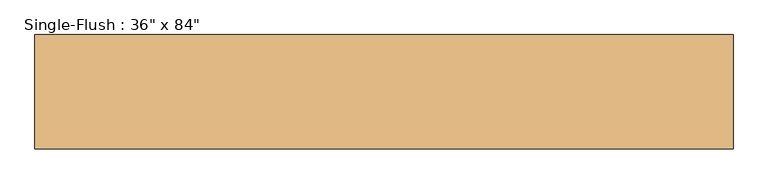
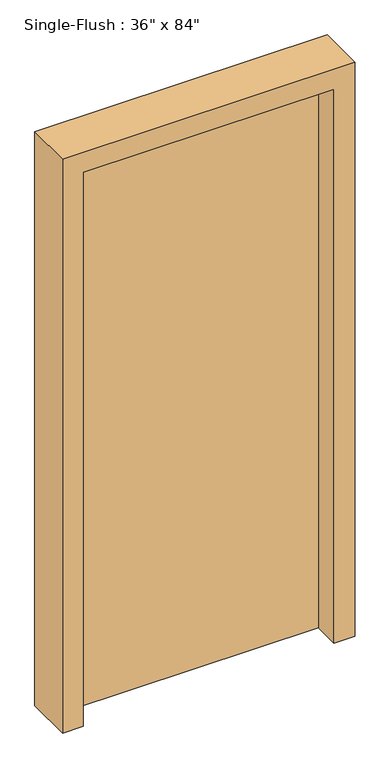
"""IFC4 building model written with IfcOpenShell, lengths in millimetres: door geometry."""

from ifc_helpers import new_model, si_unit, frame, origin, origin_with_axes, place, context, project, spatial, polyline, outline, extrude, source, transform, mapped, element, save


def door_a2dd1f53(model_context):
    return source(origin(), model_context, "Body", "SweptSolid", [
        extrude(outline(polyline([(2209.8, 533.4), (2209.8, -533.4), (0.0, -533.4), (0.0, -457.2), (2133.6, -457.2), (2133.6, 457.2), (0.0, 457.2), (0.0, 533.4), (2209.8, 533.4)])), frame((0.0, -87.3125, 0.0), z_axis=(0.0, 1.0, 0.0), x_axis=(0.0, 0.0, 1.0)), (0.0, 0.0, 1.0), 174.625),
        extrude(outline(polyline([(457.2, 11.1125), (-457.2, 11.1125), (-457.2, 61.9125), (457.2, 61.9125), (457.2, 11.1125)])), origin_with_axes(), (0.0, 0.0, 1.0), 2133.6),
    ])


if __name__ == "__main__":
    model = new_model("IFC4")
    model_context = context("Model", 3, world=origin())
    ifc_project = project(units=[si_unit("LENGTHUNIT", "METRE", prefix="MILLI")], contexts=[model_context])
    site = spatial("IfcSite", under=ifc_project)
    building = spatial("IfcBuilding", under=site)
    placement = place(None, origin())
    door_shape = door_a2dd1f53(model_context)
    element("IfcDoor", 1, ObjectType="Single-Flush : 36\" x 84\"", at=placement, inside=building, context=model_context, shape_type="MappedRepresentation", body=[
        mapped(door_shape, transform((0.0, 0.0, 0.0), x_axis=(1.0, 0.0, 0.0), y_axis=(0.0, 1.0, 0.0), z_axis=(0.0, 0.0, 1.0))),
    ])
    save(model, "model.ifc")

# Revit data of these elements
# Type "Single-Flush : 36\" x 84\""
#   Type Mark = "40"
#   Construction Type Id = "MDOOR"
#   Assembly Code = "C1020"
#   Analytic Construction = "Metal"
#   Thickness = 0' - 2"
#   Thermal Resistance (R) = 0.270117 (m²·K)/W
#   Heat Transfer Coefficient (U) = 3.7021 W/(m²·K)
#   Height = 7' - 0"
#   Trim Projection Ext = 0' - 1"
#   Trim Projection Int = 0' - 1"
#   Trim Width = 0' - 3"
#   Width = 3' - 0"
#   Door Material = Door - Panel
#   Frame Material = Door - Frame
#   Visual Light Transmittance = 0
#   Solar Heat Gain Coefficient = 0
#   Function = (empty or 0)
#   Wall Closure = (empty or 0)
# Element 1 (IfcDoor, "Single-Flush : 36\" x 84\"")
#   Materials on its faces: "Door - Frame", "Door - Panel"
# Materials
#   "Door - Panel": class "Wood", colour RGB 212 179 113, transparency 0, Cost = 0
#   "Door - Frame": class "Miscellaneous", colour RGB 65 65 65, transparency 0, Cost = 0
